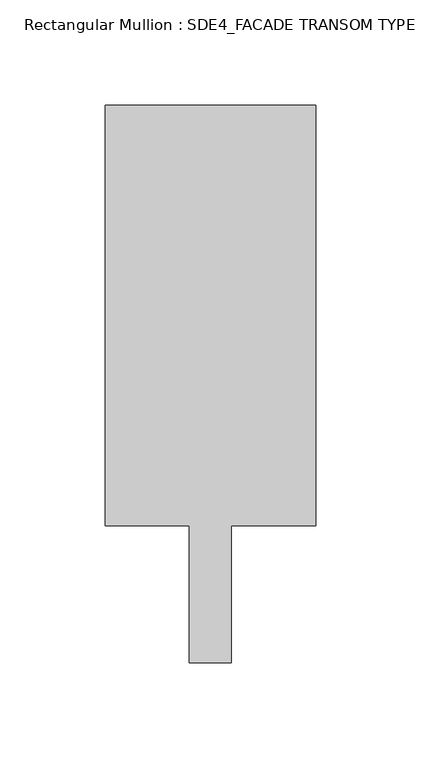
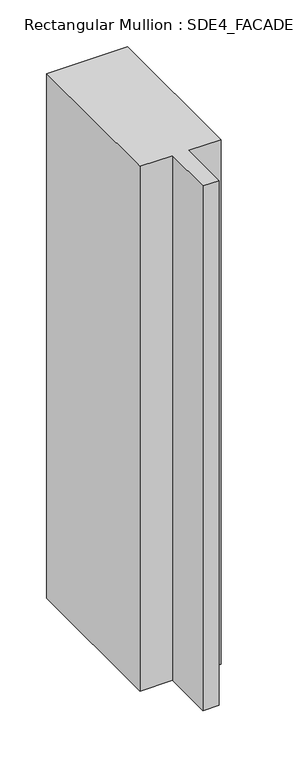
"""IFC4 building model written with IfcOpenShell, lengths in millimetres: member geometry, Rectangular Mullion : SDE4_FACADE TRANSOM TYPE 2."""

from ifc_helpers import new_model, si_unit, frame, origin, place, context, project, spatial, polyline, outline, extrude, source, transform, mapped, element, save


def rectangular_mullion_sde4_facade_transom_type_2_140d7814(model_context):
    return source(origin(), model_context, "Body", "SweptSolid", [
        extrude(outline(polyline([(50.0, 132.5), (50.0, -67.5), (10.0, -67.5), (10.0, -132.5), (-10.0, -132.5), (-10.0, -67.5), (-50.0, -67.5), (-50.0, 132.5), (50.0, 132.5)])), frame((0.0, 0.0, -684.7454401), z_axis=(0.0, 0.0, 1.0), x_axis=(1.0, 0.0, 0.0)), (0.0, 0.0, 1.0), 684.7454401),
    ])


if __name__ == "__main__":
    model = new_model("IFC4")
    model_context = context("Model", 3, world=origin())
    ifc_project = project(units=[si_unit("LENGTHUNIT", "METRE", prefix="MILLI")], contexts=[model_context])
    site = spatial("IfcSite", under=ifc_project)
    building = spatial("IfcBuilding", under=site)
    placement = place(None, origin())
    rectangular_mullion_sde4_facade_transom_type_2_shape = rectangular_mullion_sde4_facade_transom_type_2_140d7814(model_context)
    element("IfcMember", 1, ObjectType="Rectangular Mullion : SDE4_FACADE TRANSOM TYPE 2", at=placement, inside=building, context=model_context, shape_type="MappedRepresentation", body=[
        mapped(rectangular_mullion_sde4_facade_transom_type_2_shape, transform((0.0, 0.0, 0.0), x_axis=(1.0, 0.0, 0.0), y_axis=(0.0, 1.0, 0.0), z_axis=(0.0, 0.0, 1.0))),
    ])
    save(model, "model.ifc")

# Revit data of these elements
# Type "Rectangular Mullion : SDE4_FACADE TRANSOM TYPE 2"
#   built-in parameter 1007322 = 0.869423 (stored number, unit not read)
#   built-in parameter 1007321 = 0.164042 (stored number, unit not read)
#   built-in parameter 1007320 = 0.164042 (stored number, unit not read)
